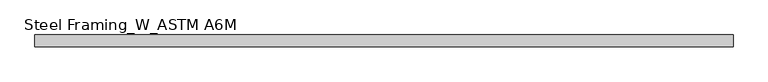
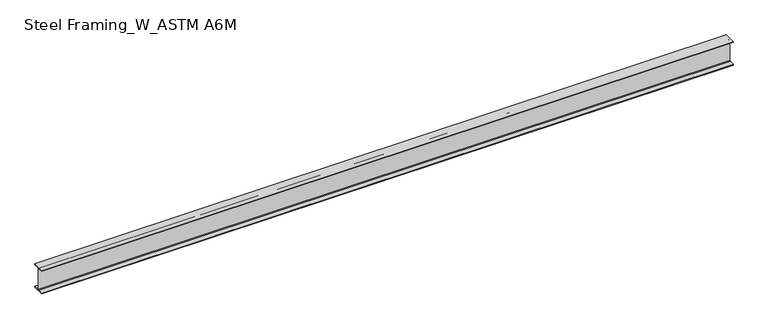
"""IFC4 building model written with IfcOpenShell, lengths in millimetres: beam geometry, Steel Framing_W_ASTM A6M : H_SB_AR_S02_W360x51_B4."""

from ifc_helpers import new_model, si_unit, point, frame, frame_2d, origin, place, context, project, spatial, polyline, circle_curve, trimmed, segment, composite_curve, outline, extrude, source, transform, mapped, element, save


def steel_framing_w_astm_a6m_e8f999e7(model_context):
    return source(origin(), model_context, "Body", "SweptSolid", [
        extrude(outline(composite_curve([segment(polyline([(85.5, -166.4), (85.5, -178.0), (-85.5, -178.0), (-85.5, -166.4), (-13.72, -166.4)]), True, "CONTINUOUS"), segment(trimmed(circle_curve(frame_2d((-13.72, -156.3)), 10.1), [point((-13.72, -166.4))], [point((-3.62, -156.3))], True, "CARTESIAN"), True, "CONTINUOUS"), segment(polyline([(-3.62, -156.3), (-3.62, 156.3)]), True, "CONTINUOUS"), segment(trimmed(circle_curve(frame_2d((-13.72, 156.3)), 10.1), [point((-3.62, 156.3))], [point((-13.72, 166.4))], True, "CARTESIAN"), True, "CONTINUOUS"), segment(polyline([(-13.72, 166.4), (-85.5, 166.4), (-85.5, 178.0), (85.5, 178.0), (85.5, 166.4), (13.72, 166.4)]), True, "CONTINUOUS"), segment(trimmed(circle_curve(frame_2d((13.72, 156.3)), 10.1), [point((13.72, 166.4))], [point((3.62, 156.3))], True, "CARTESIAN"), True, "CONTINUOUS"), segment(polyline([(3.62, 156.3), (3.62, -156.3)]), True, "CONTINUOUS"), segment(trimmed(circle_curve(frame_2d((13.72, -156.3)), 10.1), [point((3.62, -156.3))], [point((13.72, -166.4))], True, "CARTESIAN"), True, "CONTINUOUS"), segment(polyline([(13.72, -166.4), (85.5, -166.4)]), True, "CONTINUOUS")], self_intersect=False)), frame((-4987.2, 0.0, 0.0), z_axis=(1.0, 0.0, 0.0), x_axis=(0.0, 1.0, 0.0)), (0.0, 0.0, 1.0), 9974.4),
    ])


if __name__ == "__main__":
    model = new_model("IFC4")
    model_context = context("Model", 3, world=origin())
    ifc_project = project(units=[si_unit("LENGTHUNIT", "METRE", prefix="MILLI")], contexts=[model_context])
    site = spatial("IfcSite", under=ifc_project)
    building = spatial("IfcBuilding", under=site)
    placement = place(None, origin())
    steel_framing_w_astm_a6m_shape = steel_framing_w_astm_a6m_e8f999e7(model_context)
    element("IfcBeam", 1, ObjectType="Steel Framing_W_ASTM A6M : H_SB_AR_S02_W360x51_B4", at=placement, inside=building, context=model_context, shape_type="MappedRepresentation", body=[
        mapped(steel_framing_w_astm_a6m_shape, transform((0.0, 0.0, 0.0), x_axis=(1.0, 0.0, 0.0), y_axis=(0.0, 1.0, 0.0), z_axis=(0.0, 0.0, 1.0))),
    ])
    save(model, "model.ifc")

# Revit data of these elements
# Type "Steel Framing_W_ASTM A6M : H_SB_AR_S02_W360x51_B4"
#   Type Mark = "B4"
#   Section Name Key = "W14x34"
#   Width = 17.1 cm
#   Web Thickness = 0.724 cm
#   Web Fillet = 1.01 cm
#   Warping Constant = 287000.0 cm⁶
#   Torsional Moment of Inertia = 23.70 cm⁴
#   Section Area = 64.5 cm²
#   Plastic Modulus weak axis = 174.0 cm³
#   Plastic Modulus strong axis = 895.0 cm³
#   Perimeter = 1.36 m²/m
#   Nominal Weight = 51.00 kgf/m
#   Moment of Inertia weak axis = 970.00 cm⁴
#   Moment of Inertia strong axis = 14200.00 cm⁴
#   Height = 35.6 cm
#   Flange Thickness = 1.16 cm
#   Elastic Modulus weak axis = 113.0 cm³
#   Elastic Modulus strong axis = 796.0 cm³
#   Centroid Vertical = 17.8 cm
#   Centroid Horizontal = 8.55 cm
#   Length [instance default] = 1500 mm
#   Structural Material [instance default] = Steel, 45-345
#   Bolt Spacing = 0
#   Assembly Code = ""
# Element 1 (IfcBeam, "Steel Framing_W_ASTM A6M : H_SB_AR_S02_W360x51_B4")
#   Materials on its faces: "Steel, 45-345"
# Materials
#   "Steel, 45-345": class "Metal", colour RGB 189 187 185, transparency 0, Description = "Steel 345 MPa", Cost = 0
